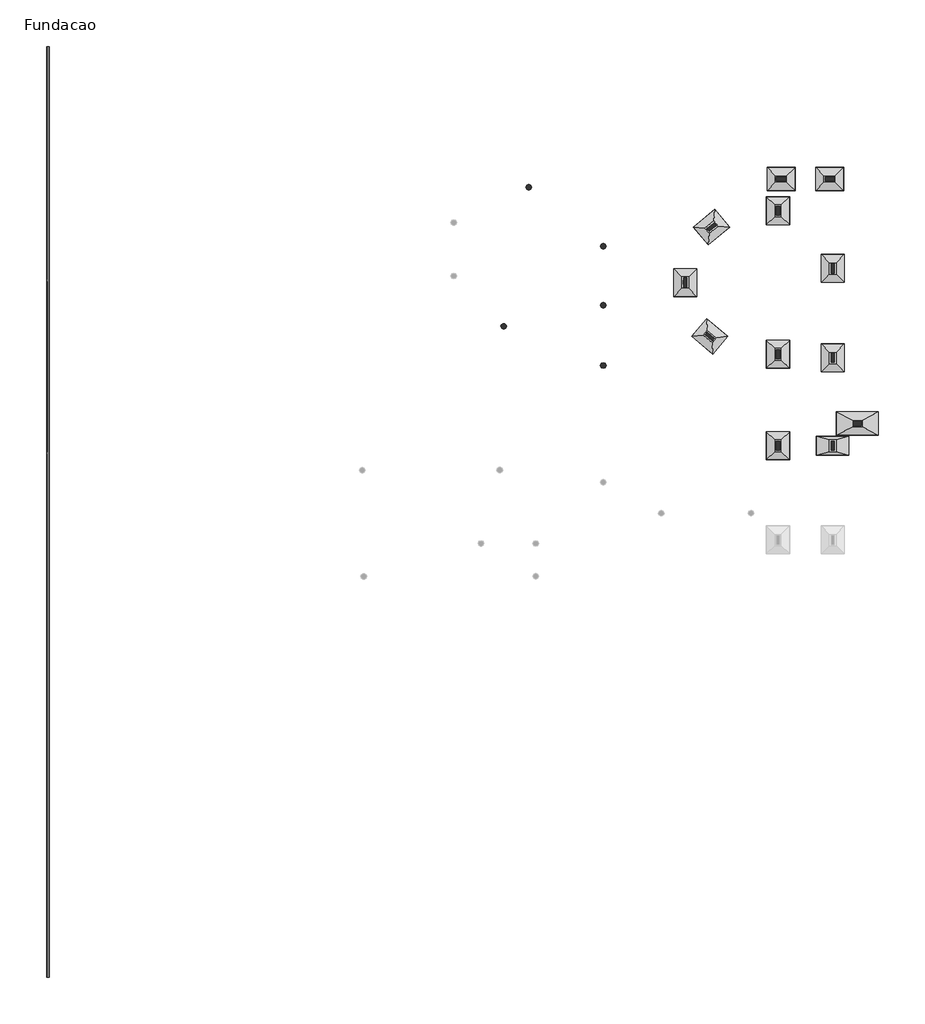
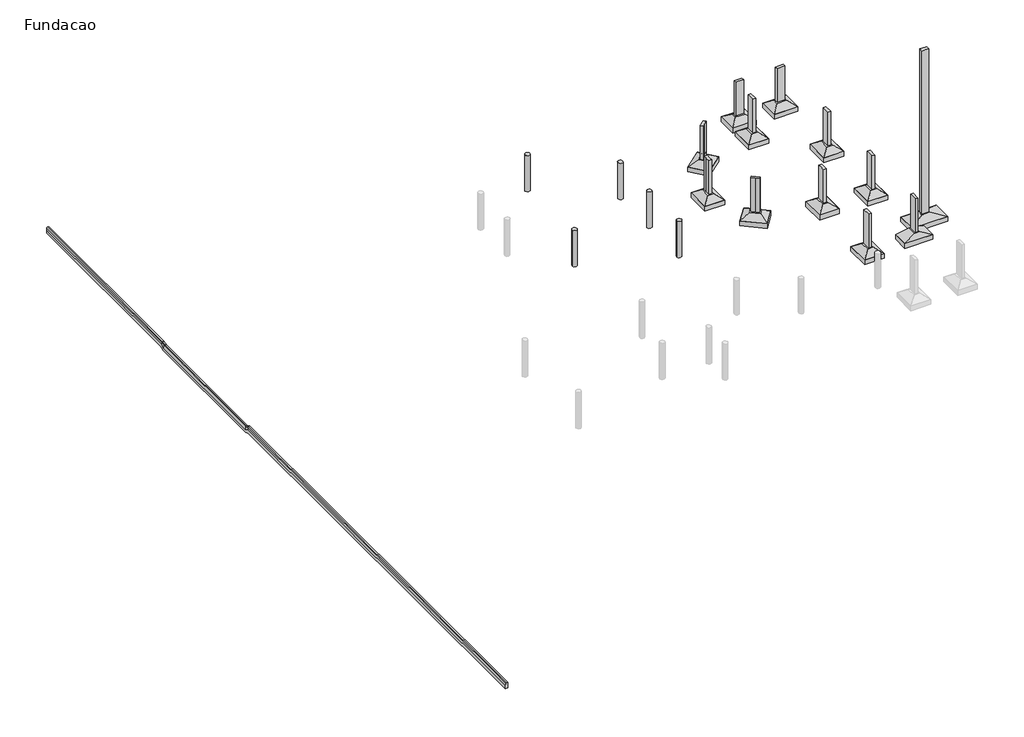
# One storey, part 2 of 2: 17 columns, 12 fasteners, 1 proxy.
"""IFC4 building model written with IfcOpenShell, lengths in millimetres."""

import ifcopenshell
import ifcopenshell.guid

model = None  # the IFC model being written
_history = None  # IfcOwnerHistory: only IFC2X3 demands one
_inside = {}  # id of a spatial element -> (the spatial element, [elements in it])
_under = {}  # id of a project, library or spatial element -> (it, [spatial elements below it])
_declared = {}  # id of a project -> (the project, [libraries it declares])
_typed = {}  # id of a type object -> (the type object, [elements of that type])
_made_of = {}  # id of a material, layer set ... -> (it, [elements and type objects made of it])


def new_model(schema):
    """Start an empty IFC model of exactly this schema.

    Asked for "IFC4X3", IfcOpenShell would pick the latest addendum, in which some entities
    have other attributes; the version numbers below select the first issue.
    IFC2X3 requires an IfcOwnerHistory on every rooted entity: one is made here for all.
    """
    global model, _history
    if schema == "IFC4X3":
        model = ifcopenshell.file(schema_version=(4, 3, 0, 0))
    else:
        model = ifcopenshell.file(schema=schema)
    _inside.clear()
    _under.clear()
    _declared.clear()
    _typed.clear()
    _made_of.clear()
    _history = None
    if model.schema == "IFC2X3":
        org = make("IfcOrganization", Name="unknown")
        user = make(
            "IfcPersonAndOrganization",
            ThePerson=make("IfcPerson", FamilyName="unknown"),
            TheOrganization=org,
        )
        app = make(
            "IfcApplication",
            ApplicationDeveloper=org,
            Version="unknown",
            ApplicationFullName="unknown",
            ApplicationIdentifier="unknown",
        )
        _history = make(
            "IfcOwnerHistory",
            OwningUser=user,
            OwningApplication=app,
            ChangeAction="ADDED",
            CreationDate=0,
        )
    return model


def make(cls, **values):
    """One entity of the class cls with the attributes given. An attribute that is None is left unset."""
    return model.create_entity(
        cls, **{name: value for name, value in values.items() if value is not None}
    )


def rooted(cls, **values):
    """An entity with a GlobalId (a new one), such as an element, a storey or a relation."""
    return make(cls, GlobalId=ifcopenshell.guid.new(), OwnerHistory=_history, **values)


def si_unit(unit_type, name, prefix=None):
    """IfcSIUnit, for example si_unit("LENGTHUNIT", "METRE", prefix="MILLI")."""
    return make("IfcSIUnit", UnitType=unit_type, Prefix=prefix, Name=name)


def assignment(units):
    """IfcUnitAssignment: the units of a project."""
    return None if units is None else make("IfcUnitAssignment", Units=units)


def point(xyz):
    """IfcCartesianPoint."""
    return None if xyz is None else make("IfcCartesianPoint", Coordinates=xyz)


def direction(xyz):
    """IfcDirection."""
    return None if xyz is None else make("IfcDirection", DirectionRatios=xyz)


def frame(location, z_axis=None, x_axis=None):
    """IfcAxis2Placement3D, a coordinate frame: its origin and axes. An axis left out is left unset."""
    return make(
        "IfcAxis2Placement3D",
        Location=point(location),
        Axis=direction(z_axis),
        RefDirection=direction(x_axis),
    )


def origin():
    """The frame at (0, 0, 0) with its axes left unset."""
    return frame((0.0, 0.0, 0.0))


def place(relative_to, where):
    """IfcLocalPlacement: puts the frame where relative to a parent placement (None: the world)."""
    return make(
        "IfcLocalPlacement", PlacementRelTo=relative_to, RelativePlacement=where
    )


def context(
    kind, dimensions, precision=None, world=None, true_north=None, identifier=None
):
    """IfcGeometricRepresentationContext, for example the 3D "Model" context."""
    return make(
        "IfcGeometricRepresentationContext",
        ContextIdentifier=identifier,
        ContextType=kind,
        CoordinateSpaceDimension=dimensions,
        Precision=precision,
        WorldCoordinateSystem=world,
        TrueNorth=true_north,
    )


def project(units=None, contexts=None):
    """IfcProject with its units and contexts."""
    return rooted(
        "IfcProject",
        Name="project",
        RepresentationContexts=contexts,
        UnitsInContext=assignment(units),
    )


def spatial(cls, under=None, at=None, **own):
    """A site, building, storey or space (cls), placed at a placement, below another one or the project."""
    s = rooted(cls, ObjectPlacement=at, **own)
    if under is not None:
        _under.setdefault(under.id(), (under, []))[1].append(s)
    return s


def polyline(points):
    """IfcPolyline through the points."""
    return make("IfcPolyline", Points=[point(p) for p in points])


def circle_curve(where, radius):
    """IfcCircle in the frame where."""
    return make("IfcCircle", Position=where, Radius=radius)


def ellipse_curve(where, semi_axis1, semi_axis2):
    """IfcEllipse in the frame where."""
    return make(
        "IfcEllipse", Position=where, SemiAxis1=semi_axis1, SemiAxis2=semi_axis2
    )


def outline(outer, holes=None, kind="AREA"):
    """IfcArbitraryClosedProfileDef: a profile drawn as a closed curve; with holes, ...WithVoids."""
    if holes is None:
        return make("IfcArbitraryClosedProfileDef", ProfileType=kind, OuterCurve=outer)
    return make(
        "IfcArbitraryProfileDefWithVoids",
        ProfileType=kind,
        OuterCurve=outer,
        InnerCurves=holes,
    )


def extrude(swept, where, along, depth):
    """IfcExtrudedAreaSolid: the profile swept, set in the frame where, extruded along a direction by depth."""
    return make(
        "IfcExtrudedAreaSolid",
        SweptArea=swept,
        Position=where,
        ExtrudedDirection=direction(along),
        Depth=depth,
    )


def faces_of(points, faces, orient=None, outer=None):
    """IfcFace entities. A face is a list of loops; a loop is a list of indices into points, from 0.

    orient and outer hold one flag for each loop. By default every Orientation is true, the
    first loop of a face is its IfcFaceOuterBound and the others are IfcFaceBound.
    """
    made = []
    for i, loops in enumerate(faces):
        bounds = []
        for j, loop in enumerate(loops):
            is_outer = j == 0 if outer is None else outer[i][j]
            bounds.append(
                make(
                    "IfcFaceOuterBound" if is_outer else "IfcFaceBound",
                    Bound=make("IfcPolyLoop", Polygon=[points[k] for k in loop]),
                    Orientation=True if orient is None else orient[i][j],
                )
            )
        made.append(make("IfcFace", Bounds=bounds))
    return made


def faceted_brep(points, faces, orient=None, outer=None, voids=None):
    """IfcFacetedBrep: a solid bounded by flat faces; with voids (closed shells), ...WithVoids."""
    shared = [point(p) for p in points]
    hull = make("IfcClosedShell", CfsFaces=faces_of(shared, faces, orient, outer))
    if voids is None:
        return make("IfcFacetedBrep", Outer=hull)
    return make(
        "IfcFacetedBrepWithVoids",
        Outer=hull,
        Voids=[
            make(cls, CfsFaces=faces_of(shared, fs, o, b)) for cls, fs, o, b in voids
        ],
    )


def shape(context_of_items, identifier, shape_type, items):
    """IfcShapeRepresentation: the items that make up one representation, for example the "Body"."""
    return make(
        "IfcShapeRepresentation",
        ContextOfItems=context_of_items,
        RepresentationIdentifier=identifier,
        RepresentationType=shape_type,
        Items=items,
    )


def source(mapping_origin, context_of_items, identifier, shape_type, items):
    """IfcRepresentationMap: a shape defined once, which mapped items show again and again."""
    return make(
        "IfcRepresentationMap",
        MappingOrigin=mapping_origin,
        MappedRepresentation=shape(context_of_items, identifier, shape_type, items),
    )


def transform(
    local_origin,
    x_axis=None,
    y_axis=None,
    z_axis=None,
    scale=None,
    scale2=None,
    scale3=None,
    uniform=True,
):
    """IfcCartesianTransformationOperator3D, or its non-uniform kind. x_axis, y_axis, z_axis: its Axis1, 2, 3."""
    if uniform:
        return make(
            "IfcCartesianTransformationOperator3D",
            Axis1=direction(x_axis),
            Axis2=direction(y_axis),
            LocalOrigin=point(local_origin),
            Scale=scale,
            Axis3=direction(z_axis),
        )
    return make(
        "IfcCartesianTransformationOperator3DnonUniform",
        Axis1=direction(x_axis),
        Axis2=direction(y_axis),
        LocalOrigin=point(local_origin),
        Scale=scale,
        Axis3=direction(z_axis),
        Scale2=scale2,
        Scale3=scale3,
    )


def mapped(mapping_source, mapping_target):
    """IfcMappedItem: shows the shape of a source again, moved by a transform."""
    return make(
        "IfcMappedItem", MappingSource=mapping_source, MappingTarget=mapping_target
    )


def made_of(thing, what):
    """Note that an element or type object is made of a material, layer set ...; save() writes the relation."""
    if what is not None:
        _made_of.setdefault(what.id(), (what, []))[1].append(thing)
    return thing


def element(
    cls,
    number,
    at=None,
    inside=None,
    cuts=None,
    type_object=None,
    material=None,
    context=None,
    identifier="Body",
    shape_type=None,
    held_by="IfcProductDefinitionShape",
    body=None,
    shapes=None,
    **own,
):
    """One element of the class cls, such as IfcWall. Its Tag is "e" and its number.

    at: its placement. inside: the storey or other place that contains it. cuts: it is an
    opening in that element (IfcRelVoidsElement). A single representation is given by context,
    identifier, shape_type and body (its items); several are given by shapes. held_by: the class
    of the entity that holds the representations. save() writes the other relations.
    """
    e = rooted(cls, Tag="e%d" % number, ObjectPlacement=at, **own)
    if body is not None:
        shapes = [shape(context, identifier, shape_type, body)]
    if shapes is not None:
        e.Representation = make(held_by, Representations=shapes)
    if inside is not None:
        _inside.setdefault(inside.id(), (inside, []))[1].append(e)
    if cuts is not None:
        rooted(
            "IfcRelVoidsElement", RelatingBuildingElement=cuts, RelatedOpeningElement=e
        )
    if type_object is not None:
        _typed.setdefault(type_object.id(), (type_object, []))[1].append(e)
    return made_of(e, material)


def aggregate(whole, parts):
    """IfcRelAggregates: a whole, such as a stair, and the parts it consists of."""
    return rooted("IfcRelAggregates", RelatingObject=whole, RelatedObjects=parts)


def save(model, path):
    """Write the relations noted so far, then the file.

    IfcRelAggregates (storeys below a building ...), IfcRelContainedInSpatialStructure (elements
    in a storey), IfcRelDefinesByType, IfcRelAssociatesMaterial and IfcRelDeclares: one each for
    every whole, place, type object, material and project.
    """
    for whole, parts in _under.values():
        aggregate(whole, parts)
    for where, things in _inside.values():
        rooted(
            "IfcRelContainedInSpatialStructure",
            RelatedElements=things,
            RelatingStructure=where,
        )
    for kind, things in _typed.values():
        rooted("IfcRelDefinesByType", RelatedObjects=things, RelatingType=kind)
    for what, things in _made_of.values():
        rooted("IfcRelAssociatesMaterial", RelatedObjects=things, RelatingMaterial=what)
    for by, libraries in _declared.values():
        rooted("IfcRelDeclares", RelatingContext=by, RelatedDefinitions=libraries)
    model.write(path)


def plane_surface(at):
    """IfcPlane: the flat surface through the origin of the frame at, square to its z axis."""
    return make("IfcPlane", Position=at)


def cylinder_surface(at, radius):
    """IfcCylindricalSurface: all points at the distance radius from the z axis of the frame at."""
    return make("IfcCylindricalSurface", Position=at, Radius=radius)


def advanced_brep(points, edges, surfaces, faces):
    """IfcAdvancedBrep: a solid bounded by faces that lie on surfaces and meet in shared edges.

    An edge is (start, end): straight between two places in points (the first is 0);
    or (start, end, curve); or (start, end, curve, False) where it runs against its curve.
    A face is (place in surfaces, loops), or (place, loops, False) where it looks against
    its surface's normal. A loop lists edges by number (the first is 1), with a minus sign
    where the edge is run from its end to its start. The first loop is the outer one.
    """
    corners = [point(p) for p in points]
    vertices = [make("IfcVertexPoint", VertexGeometry=c) for c in corners]
    made = []
    for start, end, *more in edges:
        made.append(
            make(
                "IfcEdgeCurve",
                EdgeStart=vertices[start],
                EdgeEnd=vertices[end],
                EdgeGeometry=more[0] if more else make("IfcPolyline", Points=[corners[start], corners[end]]),
                SameSense=more[1] if len(more) > 1 else True,
            )
        )
    hull = []
    for where, loops, *sense in faces:
        bounds = []
        for j, loop in enumerate(loops):
            ring = [make("IfcOrientedEdge", EdgeElement=made[abs(k) - 1], Orientation=k > 0) for k in loop]
            bounds.append(
                make(
                    "IfcFaceOuterBound" if j == 0 else "IfcFaceBound",
                    Bound=make("IfcEdgeLoop", EdgeList=ring),
                    Orientation=True,
                )
            )
        hull.append(make("IfcAdvancedFace", Bounds=bounds, FaceSurface=surfaces[where], SameSense=sense[0] if sense else True))
    return make("IfcAdvancedBrep", Outer=make("IfcClosedShell", CfsFaces=hull))


def meio_fio_meio_fio_c5939b1e(model_context):
    return source(origin(), model_context, "Body", "AdvancedBrep", [
        advanced_brep(
        [(-19460.281307, 17327.5225294, 100.0), (-19460.281307, 17327.5225294, -200.0), (-19580.281307, 17327.5225294, -200.0), (-19580.281307, 17327.5225294, -50.0), (-19560.334366, 17327.5225294, 74.7371665), (-19530.7107394, 17327.5225294, 100.0), (-19460.281307, 7304.4300153, 100.0), (-19460.281307, 7104.4300153, 20.0), (-19460.281307, 4.4300153, 20.0), (-19460.281307, -195.5699847, 100.0), (-19460.281307, -22700.938406, 100.0), (-19460.281307, -22700.938406, -200.0), (-19460.281307, -253.3447058, -200.0), (-19460.281307, -53.3447058, -280.0), (-19460.281307, 7162.2047364, -280.0), (-19460.281307, 7362.2047364, -200.0), (-19580.281307, 7362.2047364, -200.0), (-19580.281307, 7162.2047364, -280.0), (-19580.281307, -53.3447058, -280.0), (-19580.281307, -253.3447058, -200.0), (-19580.281307, -22700.938406, -200.0), (-19580.281307, -22700.938406, -50.0), (-19580.281307, -224.4573452, -50.0), (-19580.281307, -24.4573452, -130.0), (-19580.281307, 7133.3173758, -130.0), (-19580.281307, 7333.3173758, -50.0), (-19560.334366, 7309.2951925, 74.7371665), (-19530.7107394, 7304.4300153, 100.0), (-19560.334366, 7109.2951925, -5.2628335), (-19530.7107394, 7104.4300153, 20.0), (-19560.334366, -0.4351619, -5.2628335), (-19530.7107394, 4.4300153, 20.0), (-19560.334366, -200.4351619, 74.7371665), (-19530.7107394, -195.5699847, 100.0), (-19530.7107394, -22700.938406, 100.0), (-19560.334366, -22700.938406, 74.7371665)],
        [
            (0, 1),
            (1, 2),
            (2, 3),
            (3, 4),
            (4, 5, circle_curve(frame((-19530.7107394, 17327.5225294, 70.0), z_axis=(0.0, 1.0, 0.0), x_axis=(-1.0, 0.0, 0.0)), 30.0)),
            (5, 0),
            (0, 6),
            (6, 7),
            (7, 8),
            (8, 9),
            (9, 10),
            (10, 11),
            (11, 12),
            (12, 13),
            (13, 14),
            (14, 15),
            (15, 1),
            (15, 16),
            (16, 2),
            (16, 17),
            (17, 18),
            (18, 19),
            (19, 20),
            (20, 21),
            (21, 22),
            (22, 23),
            (23, 24),
            (24, 25),
            (25, 3),
            (25, 26),
            (26, 4),
            (26, 27, ellipse_curve(frame((-19530.7107394, 7310.2074874, 70.0), z_axis=(0.0, 0.9819563867314226, 0.18910752115494767), x_axis=(0.0, 0.18910752115494667, -0.9819563867314226)), 30.551255, 30.0)),
            (27, 5),
            (27, 6),
            (14, 17),
            (24, 28),
            (28, 26),
            (28, 29, ellipse_curve(frame((-19530.7107394, 7110.2074874, -10.0), z_axis=(0.0, 0.9819563867314226, 0.18910752115494764), x_axis=(0.0, -0.18910752115494842, 0.9819563867314223)), 30.551255, 30.0)),
            (29, 27),
            (29, 7),
            (13, 18),
            (23, 30),
            (30, 28),
            (30, 31, ellipse_curve(frame((-19530.7107394, -1.3474568, -10.0), z_axis=(0.0, 0.9819563867314217, -0.1891075211549513), x_axis=(0.0, 0.18910752115495252, 0.9819563867314217)), 30.551255, 30.0)),
            (31, 29),
            (31, 8),
            (12, 19),
            (22, 32),
            (32, 30),
            (32, 33, ellipse_curve(frame((-19530.7107394, -201.3474568, 70.0), z_axis=(0.0, 0.9819563867314217, -0.18910752115495139), x_axis=(0.0, -0.18910752115495078, -0.9819563867314218)), 30.551255, 30.0)),
            (33, 31),
            (33, 9),
            (10, 34),
            (34, 35, circle_curve(frame((-19530.7107394, -22700.938406, 70.0), z_axis=(0.0, -1.0, 0.0), x_axis=(-1.0, 0.0, 0.0)), 30.0)),
            (35, 21),
            (20, 11),
            (35, 32),
            (34, 33),
        ],
        [
            plane_surface(frame((-19460.281307, 17327.5225294, 100.0), z_axis=(0.0, 1.0, 0.0), x_axis=(0.0, 0.0, 1.0))),
            plane_surface(frame((-19460.281307, 17327.5225294, 100.0), z_axis=(1.0, 0.0, 0.0), x_axis=(0.0, -1.0, 0.0))),
            plane_surface(frame((-19460.281307, 17327.5225294, -200.0), z_axis=(0.0, 0.0, -1.0), x_axis=(0.0, -1.0, 0.0))),
            plane_surface(frame((-19580.281307, 17327.5225294, -200.0), z_axis=(-1.0, 0.0, 0.0), x_axis=(0.0, -1.0, 0.0))),
            plane_surface(frame((-19580.281307, 17327.5225294, -50.0), z_axis=(-0.9874542202157147, 0.0, 0.15790555081495689), x_axis=(0.0, -1.0, 0.0))),
            cylinder_surface(frame((-19530.7107394, 17327.5225294, 70.0), z_axis=(0.0, 1.0, 0.0), x_axis=(-1.0, 0.0, 0.0)), 30.0),
            plane_surface(frame((-19530.7107394, 17327.5225294, 100.0), z_axis=(0.0, 0.0, 1.0), x_axis=(0.0, -1.0, 0.0))),
            plane_surface(frame((-19460.281307, 7362.2047364, -200.0), z_axis=(0.0, 0.3713906763540969, -0.9284766908852621), x_axis=(0.0, -0.9284766908852621, -0.3713906763540969))),
            plane_surface(frame((-19580.281307, 7333.3173758, -50.0), z_axis=(-0.9874542202157147, -0.05864464931723302, 0.1466116232930858), x_axis=(0.0, -0.9284766908852622, -0.3713906763540966))),
            cylinder_surface(frame((-19530.7107394, 7315.5717356, 72.1456993), z_axis=(0.0, 0.9284766908852621, 0.3713906763540969), x_axis=(-1.0, 0.0, 0.0)), 30.0),
            plane_surface(frame((-19530.7107394, 7304.4300153, 100.0), z_axis=(0.0, -0.37139067635409667, 0.9284766908852622), x_axis=(0.0, -0.9284766908852622, -0.37139067635409667))),
            plane_surface(frame((-19460.281307, 7162.2047364, -280.0), z_axis=(0.0, 0.0, -1.0), x_axis=(0.0, -1.0, 0.0))),
            plane_surface(frame((-19580.281307, 7133.3173758, -130.0), z_axis=(-0.9874542202157146, 0.0, 0.15790555081495686), x_axis=(0.0, -1.0, 0.0))),
            cylinder_surface(frame((-19530.7107394, 7104.4300153, -10.0), z_axis=(0.0, 1.0, 0.0), x_axis=(-1.0, 0.0, 0.0)), 30.0),
            plane_surface(frame((-19530.7107394, 7104.4300153, 20.0), z_axis=(0.0, 0.0, 1.0), x_axis=(0.0, -1.0, 0.0))),
            plane_surface(frame((-19460.281307, -53.3447058, -280.0), z_axis=(0.0, -0.37139067635410367, -0.9284766908852594), x_axis=(0.0, -0.9284766908852594, 0.37139067635410367))),
            plane_surface(frame((-19580.281307, -24.4573452, -130.0), z_axis=(-0.9874542202157147, 0.05864464931723411, 0.14661162329308536), x_axis=(0.0, -0.9284766908852594, 0.37139067635410355))),
            cylinder_surface(frame((-19530.7107394, -6.711705, -7.8543007), z_axis=(0.0, 0.9284766908852593, -0.3713906763541038), x_axis=(-1.0, 0.0, 0.0)), 30.0),
            plane_surface(frame((-19530.7107394, 4.4300153, 20.0), z_axis=(0.0, 0.3713906763541038, 0.9284766908852593), x_axis=(0.0, -0.9284766908852593, 0.3713906763541038))),
            plane_surface(frame((-19460.281307, -22700.938406, 100.0), z_axis=(0.0, -1.0, 0.0), x_axis=(0.0, 0.0, 1.0))),
            plane_surface(frame((-19460.281307, -253.3447058, -200.0), z_axis=(0.0, 0.0, -1.0), x_axis=(0.0, -1.0, 0.0))),
            plane_surface(frame((-19580.281307, -224.4573452, -50.0), z_axis=(-0.9874542202157146, 0.0, 0.15790555081495683), x_axis=(0.0, -1.0, 0.0))),
            cylinder_surface(frame((-19530.7107394, -195.5699847, 70.0), z_axis=(0.0, 1.0, 0.0), x_axis=(-1.0, 0.0, 0.0)), 30.0),
            plane_surface(frame((-19530.7107394, -195.5699847, 100.0), z_axis=(0.0, 0.0, 1.0), x_axis=(0.0, -1.0, 0.0))),
        ],
        [
            (0, [[1, 2, 3, 4, 5, 6]]),
            (1, [[-1, 7, 8, 9, 10, 11, 12, 13, 14, 15, 16, 17]]),
            (2, [[-2, -17, 18, 19]]),
            (3, [[-3, -19, 20, 21, 22, 23, 24, 25, 26, 27, 28, 29]]),
            (4, [[-4, -29, 30, 31]]),
            (5, [[-5, -31, 32, 33]]),
            (6, [[-6, -33, 34, -7]]),
            (7, [[-18, -16, 35, -20]]),
            (8, [[-30, -28, 36, 37]]),
            (9, [[-32, -37, 38, 39]]),
            (10, [[-34, -39, 40, -8]]),
            (11, [[-35, -15, 41, -21]]),
            (12, [[-36, -27, 42, 43]]),
            (13, [[-38, -43, 44, 45]]),
            (14, [[-40, -45, 46, -9]]),
            (15, [[-41, -14, 47, -22]]),
            (16, [[-42, -26, 48, 49]]),
            (17, [[-44, -49, 50, 51]]),
            (18, [[-46, -51, 52, -10]]),
            (19, [[53, 54, 55, -24, 56, -12]]),
            (20, [[-47, -13, -56, -23]]),
            (21, [[-48, -25, -55, 57]]),
            (22, [[-50, -57, -54, 58]]),
            (23, [[-52, -58, -53, -11]]),
        ],
    ),
    ])


def s14_8166d2be(model_context):
    return source(origin(), model_context, "Body", "SolidModel", [
        faceted_brep([(-55.0, 0.0, 0.0), (-345.0, 0.0, 0.0), (-345.0, -400.0, 0.0), (-55.0, -400.0, 0.0), (300.0, 700.0, -250.0), (300.0, -1100.0, -250.0), (-700.0, -1100.0, -250.0), (-700.0, 700.0, -250.0)], [[[0, 1, 2, 3]], [[4, 5, 6, 7]], [[4, 7, 1, 0]], [[7, 6, 2, 1]], [[6, 5, 3, 2]], [[5, 4, 0, 3]]]),
        extrude(outline(polyline([(300.0, 700.0), (300.0, -1100.0), (-700.0, -1100.0), (-700.0, 700.0), (300.0, 700.0)])), frame((0.0, 0.0, -500.0), z_axis=(0.0, 0.0, 1.0), x_axis=(1.0, 0.0, 0.0)), (0.0, 0.0, 1.0), 250.0),
    ])


def sps1_6b3be553(model_context):
    return source(origin(), model_context, "Body", "SolidModel", [
        faceted_brep([(-55.0, 50.0, 0.0), (-345.0, 50.0, 0.0), (-345.0, -450.0, 0.0), (-55.0, -450.0, 0.0), (300.0, 400.0, -250.0), (300.0, -800.0, -250.0), (-700.0, -800.0, -250.0), (-700.0, 400.0, -250.0)], [[[0, 1, 2, 3]], [[4, 5, 6, 7]], [[4, 7, 1, 0]], [[7, 6, 2, 1]], [[6, 5, 3, 2]], [[5, 4, 0, 3]]]),
        extrude(outline(polyline([(300.0, 400.0), (300.0, -800.0), (-700.0, -800.0), (-700.0, 400.0), (300.0, 400.0)])), frame((0.0, 0.0, -500.0), z_axis=(0.0, 0.0, 1.0), x_axis=(1.0, 0.0, 0.0)), (0.0, 0.0, 1.0), 250.0),
    ])


def sps11_3ae28187(model_context):
    return source(origin(), model_context, "Body", "SolidModel", [
        faceted_brep([(-55.0, 50.0, 0.0), (-345.0, 50.0, 0.0), (-345.0, -450.0, 0.0), (-55.0, -450.0, 0.0), (500.0, 200.0, -250.0), (500.0, -600.0, -250.0), (-900.0, -600.0, -250.0), (-900.0, 200.0, -250.0)], [[[0, 1, 2, 3]], [[4, 5, 6, 7]], [[4, 7, 1, 0]], [[7, 6, 2, 1]], [[6, 5, 3, 2]], [[5, 4, 0, 3]]]),
        extrude(outline(polyline([(500.0, 200.0), (500.0, -600.0), (-900.0, -600.0), (-900.0, 200.0), (500.0, 200.0)])), frame((0.0, 0.0, -500.0), z_axis=(0.0, 0.0, 1.0), x_axis=(1.0, 0.0, 0.0)), (0.0, 0.0, 1.0), 250.0),
    ])


model = new_model("IFC4")

# Units and contexts
model_context = context("Model", 3, world=origin())
ifc_project = project(units=[si_unit("LENGTHUNIT", "METRE", prefix="MILLI")], contexts=[model_context])

# Site, building, storey
site = spatial("IfcSite", under=ifc_project)
building = spatial("IfcBuilding", under=site)
storey = spatial("IfcBuildingStorey", under=building, Name="Fundacao", Elevation=-1200.0)

# Proxy
placement = place(None, origin())
meio_fio_meio_fio_shape = meio_fio_meio_fio_c5939b1e(model_context)
element("IfcBuildingElementProxy", 1, Name="MEIO-FIO : MEIO-FIO", ObjectType="MEIO-FIO : MEIO-FIO", at=placement, inside=storey, context=model_context, shape_type="MappedRepresentation", body=[
    mapped(meio_fio_meio_fio_shape, transform((0.0, 0.0, 0.0), x_axis=(1.0, 0.0, 0.0), y_axis=(0.0, 1.0, 0.0), z_axis=(0.0, 0.0, 1.0))),
])

# Columns
element("IfcColumn", 2, ObjectType="TQS - Pilar circular : TQS - Pilar circular 25.0cm", at=placement, inside=storey, context=model_context, shape_type="AdvancedBrep", body=[
    advanced_brep(
    [(-51.2, 5294.463685, -1500.0), (198.8, 5294.463685, -1500.0), (-51.2, 5294.463685, 430.0), (198.8, 5294.463685, 430.0), (143.8, 5190.9021092, 430.0), (3.8, 5190.9021092, 430.0)],
    [
        (0, 1, circle_curve(frame((73.8, 5294.463685, -1500.0), z_axis=(0.0, 0.0, -1.0), x_axis=(1.0, 0.0, 0.0)), 125.0)),
        (1, 0, circle_curve(frame((73.8, 5294.463685, -1500.0), z_axis=(0.0, 0.0, -1.0), x_axis=(1.0, 0.0, 0.0)), 125.0)),
        (2, 3, circle_curve(frame((73.8, 5294.463685, 430.0), z_axis=(0.0, 0.0, -1.0), x_axis=(1.0, 0.0, 0.0)), 125.0)),
        (3, 1),
        (0, 2),
        (3, 4, circle_curve(frame((73.8, 5294.463685, 430.0), z_axis=(0.0, 0.0, -1.0), x_axis=(1.0, 0.0, 0.0)), 125.0)),
        (4, 5, circle_curve(frame((73.8, 5294.463685, 430.0), z_axis=(0.0, 0.0, -1.0), x_axis=(1.0, 0.0, 0.0)), 125.0)),
        (5, 2, circle_curve(frame((73.8, 5294.463685, 430.0), z_axis=(0.0, 0.0, -1.0), x_axis=(1.0, 0.0, 0.0)), 125.0)),
    ],
    [
        plane_surface(frame((198.8, 5294.463685, -1500.0), z_axis=(0.0, 0.0, -1.0), x_axis=(0.0, -1.0, 0.0))),
        cylinder_surface(frame((73.8, 5294.463685, -1500.0), z_axis=(0.0, 0.0, 1.0), x_axis=(1.0, 0.0, 0.0)), 125.0),
        plane_surface(frame((198.8, 5294.463685, 430.0), z_axis=(0.0, 0.0, 1.0), x_axis=(0.0, 1.0, 0.0))),
    ],
    [
        (0, [[1, 2]]),
        (1, [[3, 4, -1, 5]]),
        (1, [[6, 7, 8, -5, -2, -4]]),
        (2, [[-8, -7, -6, -3]]),
    ],
),
])
element("IfcColumn", 3, ObjectType="TQS - Pilar circular : TQS - Pilar circular 25.0cm", at=placement, inside=storey, context=model_context, shape_type="AdvancedBrep", body=[
    advanced_brep(
    [(1025.0, 11273.8, -1500.0), (1275.0, 11273.8, -1500.0), (1025.0, 11273.8, 430.0), (1068.781362, 11368.818592, 430.0), (1231.240384, 11368.8, 430.0), (1275.0, 11273.8, 430.0), (1231.240384, 11178.8, 430.0), (1068.781362, 11178.781408, 430.0)],
    [
        (0, 1, circle_curve(frame((1150.0, 11273.8, -1500.0), z_axis=(0.0, 0.0, -1.0), x_axis=(1.0, 0.0, 0.0)), 125.0)),
        (1, 0, circle_curve(frame((1150.0, 11273.8, -1500.0), z_axis=(0.0, 0.0, -1.0), x_axis=(1.0, 0.0, 0.0)), 125.0)),
        (2, 3, circle_curve(frame((1150.0, 11273.8, 430.0), z_axis=(0.0, 0.0, -1.0), x_axis=(1.0, 0.0, 0.0)), 125.0)),
        (3, 4, circle_curve(frame((1150.0, 11273.8, 430.0), z_axis=(0.0, 0.0, -1.0), x_axis=(1.0, 0.0, 0.0)), 125.0)),
        (4, 5, circle_curve(frame((1150.0, 11273.8, 430.0), z_axis=(0.0, 0.0, -1.0), x_axis=(1.0, 0.0, 0.0)), 125.0)),
        (5, 1),
        (0, 2),
        (5, 6, circle_curve(frame((1150.0, 11273.8, 430.0), z_axis=(0.0, 0.0, -1.0), x_axis=(1.0, 0.0, 0.0)), 125.0)),
        (6, 7, circle_curve(frame((1150.0, 11273.8, 430.0), z_axis=(0.0, 0.0, -1.0), x_axis=(1.0, 0.0, 0.0)), 125.0)),
        (7, 2, circle_curve(frame((1150.0, 11273.8, 430.0), z_axis=(0.0, 0.0, -1.0), x_axis=(1.0, 0.0, 0.0)), 125.0)),
    ],
    [
        plane_surface(frame((1275.0, 11273.8, -1500.0), z_axis=(0.0, 0.0, -1.0), x_axis=(0.0, -1.0, 0.0))),
        cylinder_surface(frame((1150.0, 11273.8, -1500.0), z_axis=(0.0, 0.0, 1.0), x_axis=(1.0, 0.0, 0.0)), 125.0),
        plane_surface(frame((1275.0, 11273.8, 430.0), z_axis=(0.0, 0.0, 1.0), x_axis=(0.0, 1.0, 0.0))),
    ],
    [
        (0, [[1, 2]]),
        (1, [[3, 4, 5, 6, -1, 7]]),
        (1, [[8, 9, 10, -7, -2, -6]]),
        (2, [[-10, -9, -8, -5, -4, -3]]),
    ],
),
])
element("IfcColumn", 4, ObjectType="TQS - Pilar circular : TQS - Pilar circular 25.0cm", at=placement, inside=storey, context=model_context, shape_type="AdvancedBrep", body=[
    advanced_brep(
    [(4239.0, 6198.7999999, -1500.0), (4489.0, 6198.7999999, -1500.0), (4239.0, 6198.7999999, 430.0), (4269.0, 6280.040384, 430.0), (4459.0, 6280.040384, 430.0), (4489.0, 6198.7999999, 430.0), (4459.0, 6117.5596159, 430.0), (4269.0, 6117.5596159, 430.0)],
    [
        (0, 1, circle_curve(frame((4364.0, 6198.7999999, -1500.0), z_axis=(0.0, 0.0, -1.0), x_axis=(1.0, 0.0, 0.0)), 125.0)),
        (1, 0, circle_curve(frame((4364.0, 6198.7999999, -1500.0), z_axis=(0.0, 0.0, -1.0), x_axis=(1.0, 0.0, 0.0)), 125.0)),
        (2, 3, circle_curve(frame((4364.0, 6198.7999999, 430.0), z_axis=(0.0, 0.0, -1.0), x_axis=(1.0, 0.0, 0.0)), 125.0)),
        (3, 4, circle_curve(frame((4364.0, 6198.7999999, 430.0), z_axis=(0.0, 0.0, -1.0), x_axis=(1.0, 0.0, 0.0)), 125.0)),
        (4, 5, circle_curve(frame((4364.0, 6198.7999999, 430.0), z_axis=(0.0, 0.0, -1.0), x_axis=(1.0, 0.0, 0.0)), 125.0)),
        (5, 1),
        (0, 2),
        (5, 6, circle_curve(frame((4364.0, 6198.7999999, 430.0), z_axis=(0.0, 0.0, -1.0), x_axis=(1.0, 0.0, 0.0)), 125.0)),
        (6, 7, circle_curve(frame((4364.0, 6198.7999999, 430.0), z_axis=(0.0, 0.0, -1.0), x_axis=(1.0, 0.0, 0.0)), 125.0)),
        (7, 2, circle_curve(frame((4364.0, 6198.7999999, 430.0), z_axis=(0.0, 0.0, -1.0), x_axis=(1.0, 0.0, 0.0)), 125.0)),
    ],
    [
        plane_surface(frame((4489.0, 6198.7999999, -1500.0), z_axis=(0.0, 0.0, -1.0), x_axis=(0.0, -1.0, 0.0))),
        cylinder_surface(frame((4364.0, 6198.7999999, -1500.0), z_axis=(0.0, 0.0, 1.0), x_axis=(1.0, 0.0, 0.0)), 125.0),
        plane_surface(frame((4489.0, 6198.7999999, 430.0), z_axis=(0.0, 0.0, 1.0), x_axis=(0.0, 1.0, 0.0))),
    ],
    [
        (0, [[1, 2]]),
        (1, [[3, 4, 5, 6, -1, 7]]),
        (1, [[8, 9, 10, -7, -2, -6]]),
        (2, [[-10, -9, -8, -5, -4, -3]]),
    ],
),
])
element("IfcColumn", 5, ObjectType="TQS - Pilar circular : TQS - Pilar circular 25.0cm", at=placement, inside=storey, context=model_context, shape_type="AdvancedBrep", body=[
    advanced_brep(
    [(4239.0, 8736.2999999, -1500.0), (4489.0, 8736.2999999, -1500.0), (4239.0, 8736.2999999, 430.0), (4269.0, 8817.540384, 430.0), (4459.0, 8817.540384, 430.0), (4489.0, 8736.2999999, 430.0), (4459.0, 8655.0596159, 430.0), (4269.0, 8655.0596159, 430.0)],
    [
        (0, 1, circle_curve(frame((4364.0, 8736.2999999, -1500.0), z_axis=(0.0, 0.0, -1.0), x_axis=(1.0, 0.0, 0.0)), 125.0)),
        (1, 0, circle_curve(frame((4364.0, 8736.2999999, -1500.0), z_axis=(0.0, 0.0, -1.0), x_axis=(1.0, 0.0, 0.0)), 125.0)),
        (2, 3, circle_curve(frame((4364.0, 8736.2999999, 430.0), z_axis=(0.0, 0.0, -1.0), x_axis=(1.0, 0.0, 0.0)), 125.0)),
        (3, 4, circle_curve(frame((4364.0, 8736.2999999, 430.0), z_axis=(0.0, 0.0, -1.0), x_axis=(1.0, 0.0, 0.0)), 125.0)),
        (4, 5, circle_curve(frame((4364.0, 8736.2999999, 430.0), z_axis=(0.0, 0.0, -1.0), x_axis=(1.0, 0.0, 0.0)), 125.0)),
        (5, 1),
        (0, 2),
        (5, 6, circle_curve(frame((4364.0, 8736.2999999, 430.0), z_axis=(0.0, 0.0, -1.0), x_axis=(1.0, 0.0, 0.0)), 125.0)),
        (6, 7, circle_curve(frame((4364.0, 8736.2999999, 430.0), z_axis=(0.0, 0.0, -1.0), x_axis=(1.0, 0.0, 0.0)), 125.0)),
        (7, 2, circle_curve(frame((4364.0, 8736.2999999, 430.0), z_axis=(0.0, 0.0, -1.0), x_axis=(1.0, 0.0, 0.0)), 125.0)),
    ],
    [
        plane_surface(frame((4489.0, 8736.2999999, -1500.0), z_axis=(0.0, 0.0, -1.0), x_axis=(0.0, -1.0, 0.0))),
        cylinder_surface(frame((4364.0, 8736.2999999, -1500.0), z_axis=(0.0, 0.0, 1.0), x_axis=(1.0, 0.0, 0.0)), 125.0),
        plane_surface(frame((4489.0, 8736.2999999, 430.0), z_axis=(0.0, 0.0, 1.0), x_axis=(0.0, 1.0, 0.0))),
    ],
    [
        (0, [[1, 2]]),
        (1, [[3, 4, 5, 6, -1, 7]]),
        (1, [[8, 9, 10, -7, -2, -6]]),
        (2, [[-10, -9, -8, -5, -4, -3]]),
    ],
),
])
element("IfcColumn", 6, ObjectType="TQS - Pilar circular : TQS - Pilar circular 25.0cm", at=placement, inside=storey, context=model_context, shape_type="AdvancedBrep", body=[
    advanced_brep(
    [(4239.0, 3610.8, -1500.0), (4489.0, 3610.8, -1500.0), (4239.0, 3610.8, 430.0), (4269.0, 3692.040384, 430.0), (4459.0, 3692.040384, 430.0), (4489.0, 3610.8, 430.0), (4459.0, 3529.5596159, 430.0), (4269.0, 3529.5596159, 430.0)],
    [
        (0, 1, circle_curve(frame((4364.0, 3610.8, -1500.0), z_axis=(0.0, 0.0, -1.0), x_axis=(1.0, 0.0, 0.0)), 125.0)),
        (1, 0, circle_curve(frame((4364.0, 3610.8, -1500.0), z_axis=(0.0, 0.0, -1.0), x_axis=(1.0, 0.0, 0.0)), 125.0)),
        (2, 3, circle_curve(frame((4364.0, 3610.8, 430.0), z_axis=(0.0, 0.0, -1.0), x_axis=(1.0, 0.0, 0.0)), 125.0)),
        (3, 4, circle_curve(frame((4364.0, 3610.8, 430.0), z_axis=(0.0, 0.0, -1.0), x_axis=(1.0, 0.0, 0.0)), 125.0)),
        (4, 5, circle_curve(frame((4364.0, 3610.8, 430.0), z_axis=(0.0, 0.0, -1.0), x_axis=(1.0, 0.0, 0.0)), 125.0)),
        (5, 1),
        (0, 2),
        (5, 6, circle_curve(frame((4364.0, 3610.8, 430.0), z_axis=(0.0, 0.0, -1.0), x_axis=(1.0, 0.0, 0.0)), 125.0)),
        (6, 7, circle_curve(frame((4364.0, 3610.8, 430.0), z_axis=(0.0, 0.0, -1.0), x_axis=(1.0, 0.0, 0.0)), 125.0)),
        (7, 2, circle_curve(frame((4364.0, 3610.8, 430.0), z_axis=(0.0, 0.0, -1.0), x_axis=(1.0, 0.0, 0.0)), 125.0)),
    ],
    [
        plane_surface(frame((4489.0, 3610.8, -1500.0), z_axis=(0.0, 0.0, -1.0), x_axis=(0.0, -1.0, 0.0))),
        cylinder_surface(frame((4364.0, 3610.8, -1500.0), z_axis=(0.0, 0.0, 1.0), x_axis=(1.0, 0.0, 0.0)), 125.0),
        plane_surface(frame((4489.0, 3610.8, 430.0), z_axis=(0.0, 0.0, 1.0), x_axis=(0.0, 1.0, 0.0))),
    ],
    [
        (0, [[1, 2]]),
        (1, [[3, 4, 5, 6, -1, 7]]),
        (1, [[8, 9, 10, -7, -2, -6]]),
        (2, [[-10, -9, -8, -5, -4, -3]]),
    ],
),
])
element("IfcColumn", 7, ObjectType="TQS - Pilar retangular : 14.0 x 40.0", at=placement, inside=storey, context=model_context, shape_type="Brep", body=[
    faceted_brep([(14294.0, 11563.8, -1450.0), (14154.0, 11563.8, -1450.0), (13894.0, 11563.8, -1450.0), (13894.0, 11703.8, -1450.0), (14294.0, 11703.8, -1450.0), (14294.0, 11563.8, 350.0), (14154.0, 11563.8, 350.0), (13894.0, 11563.8, 350.0), (13894.0, 11703.8, 350.0), (14294.0, 11703.8, 350.0)], [[[0, 1, 2, 3, 4]], [[5, 6, 7, 2, 1, 0]], [[7, 8, 3, 2]], [[8, 9, 4, 3]], [[9, 5, 0, 4]], [[5, 9, 8, 7, 6]]]),
])
element("IfcColumn", 8, ObjectType="TQS - Pilar retangular : 14.0 x 40.0", at=placement, inside=storey, context=model_context, shape_type="Brep", body=[
    faceted_brep([(12206.0, 11563.8, -1450.0), (11946.0031341, 11563.8, -1450.0), (11806.0, 11563.8, -1450.0), (11806.0, 11703.8, -1450.0), (12206.0, 11703.8, -1450.0), (12206.0, 11563.8, 350.0), (11946.0031341, 11563.8, 350.0), (11806.0, 11563.8, 350.0), (11806.0, 11703.8, 350.0), (12206.0, 11703.8, 350.0)], [[[0, 1, 2, 3, 4]], [[5, 6, 7, 2, 1, 0]], [[7, 8, 3, 2]], [[8, 9, 4, 3]], [[9, 5, 0, 4]], [[5, 9, 8, 7, 6]]]),
])
element("IfcColumn", 9, ObjectType="TQS - Pilar retangular : 14.0 x 40.0", at=placement, inside=storey, context=model_context, shape_type="Brep", body=[
    faceted_brep([(11806.0031341, 10065.0703526, -1450.0), (11806.0031341, 10209.2668795, -1450.0), (11806.0031341, 10465.0703526, -1450.0), (11946.0031341, 10465.0703526, -1450.0), (11946.0031341, 10065.0703526, -1450.0), (11806.0031341, 10065.0703526, -1250.0), (11806.0031341, 10065.0703526, 350.0), (11806.0031341, 10209.2668795, 350.0), (11806.0031341, 10465.0703526, 350.0), (11946.0031341, 10465.0703526, 350.0), (11946.0031341, 10465.0703526, -1250.0), (11946.0031341, 10065.0703526, 350.0), (11946.0031341, 10065.0703526, -1250.0)], [[[0, 1, 2, 3, 4]], [[2, 1, 0, 5, 6, 7, 8]], [[3, 2, 8, 9, 10]], [[4, 3, 10, 9, 11, 12]], [[0, 4, 12, 11, 6, 5]], [[8, 7, 6, 11, 9]]]),
])
element("IfcColumn", 10, ObjectType="TQS - Pilar retangular : 14.0 x 40.0", at=placement, inside=storey, context=model_context, shape_type="Brep", body=[
    faceted_brep([(11806.0, 3898.2763649, -1450.0), (11806.0, 4154.0974781, -1450.0), (11806.0, 4298.2763649, -1450.0), (11946.0, 4298.2763649, -1450.0), (11946.0, 3898.2763649, -1450.0), (11806.0, 3898.2763649, 350.0), (11806.0, 4154.0974781, 350.0), (11806.0, 4298.2763649, 350.0), (11806.0, 4298.2763649, -1250.0), (11946.0, 4298.2763649, 350.0), (11946.0, 4298.2763649, -1250.0), (11946.0, 3898.2763649, 350.0), (11946.0, 3898.2763649, -1250.0)], [[[0, 1, 2, 3, 4]], [[2, 1, 0, 5, 6, 7, 8]], [[3, 2, 8, 7, 9, 10]], [[4, 3, 10, 9, 11, 12]], [[0, 4, 12, 11, 5]], [[7, 6, 5, 11, 9]]]),
])
element("IfcColumn", 11, ObjectType="TQS - Pilar retangular : 14.0 x 40.0", at=placement, inside=storey, context=model_context, shape_type="Brep", body=[
    faceted_brep([(11806.0, -35.7794604, -1450.0), (11806.0, 364.2205396, -1450.0), (11946.0, 364.2205396, -1450.0), (11946.0, -35.7794604, -1450.0), (11806.0, -35.7794604, 350.0), (11806.0, 364.2205396, 350.0), (11946.0, 364.2205396, 350.0), (11946.0, 364.2205396, -1250.0), (11946.0, -35.7794604, 350.0), (11946.0, -35.7794604, -1250.0)], [[[0, 1, 2, 3]], [[1, 0, 4, 5]], [[2, 1, 5, 6, 7]], [[3, 2, 7, 6, 8, 9]], [[0, 3, 9, 8, 4]], [[5, 4, 8, 6]]]),
])
element("IfcColumn", 12, ObjectType="TQS - Pilar retangular : 14.0 x 40.0", at=placement, inside=storey, context=model_context, shape_type="SweptSolid", body=[
    extrude(outline(polyline([(14154.0, -35.7794604), (14154.0, 364.2205396), (14294.0, 364.2205396), (14294.0, -35.7794604), (14154.0, -35.7794604)])), frame((0.0, 0.0, -1450.0), z_axis=(0.0, 0.0, 1.0), x_axis=(1.0, 0.0, 0.0)), (0.0, 0.0, 1.0), 1800.0),
])
element("IfcColumn", 13, ObjectType="TQS - Pilar retangular : 14.0 x 40.0", at=placement, inside=storey, context=model_context, shape_type="SweptSolid", body=[
    extrude(outline(polyline([(14154.0, 3742.9688701), (14154.0, 4142.9688701), (14294.0, 4142.9688701), (14294.0, 3742.9688701), (14154.0, 3742.9688701)])), frame((0.0, 0.0, -1450.0), z_axis=(0.0, 0.0, 1.0), x_axis=(1.0, 0.0, 0.0)), (0.0, 0.0, 1.0), 1800.0),
])
element("IfcColumn", 14, ObjectType="TQS - Pilar retangular : 14.0 x 40.0", at=placement, inside=storey, context=model_context, shape_type="SweptSolid", body=[
    extrude(outline(polyline([(14154.0, 7588.3844351), (14154.0, 7988.3844351), (14294.0, 7988.3844351), (14294.0, 7588.3844351), (14154.0, 7588.3844351)])), frame((0.0, 0.0, -1450.0), z_axis=(0.0, 0.0, 1.0), x_axis=(1.0, 0.0, 0.0)), (0.0, 0.0, 1.0), 1800.0),
])
element("IfcColumn", 15, ObjectType="TQS - Pilar retangular : 19.0 x 35.0", at=placement, inside=storey, context=model_context, shape_type="Brep", body=[
    faceted_brep([(15109.0, 1218.8, -1450.0), (15459.0, 1218.8, -1450.0), (15459.0, 1028.8, -1450.0), (15109.0, 1028.8, -1450.0), (15109.0, 1218.8, 7250.0), (15459.0, 1218.8, 7250.0), (15109.0, 1218.8, 3030.0), (15109.0, 1218.8, 3530.0), (15459.0, 1028.8, 7250.0), (15459.0, 1028.8, 6450.0), (15459.0, 1028.8, 3530.0), (15459.0, 1028.8, 3030.0), (15269.0, 1028.8, 7250.0), (15109.0, 1028.8, 7250.0), (15109.0, 1028.8, 3530.0), (15109.0, 1028.8, 3030.0)], [[[0, 1, 2, 3]], [[4, 5, 1, 0, 6, 7]], [[5, 8, 9, 10, 11, 2, 1]], [[8, 12, 13, 14, 15, 3, 2, 11, 10, 9]], [[13, 4, 7, 6, 0, 3, 15, 14]], [[4, 13, 12, 8, 5]]]),
])
element("IfcColumn", 16, ObjectType="TQS - Pilar Polig_1 : TQS Column", at=placement, inside=storey, context=model_context, shape_type="Brep", body=[
    faceted_brep([(8972.0852614, 9622.0701515, -1450.0), (8976.3671199, 9625.3602237, -1450.0), (9127.4604175, 9741.4565052, -1450.0), (9213.935877, 9632.7302414, -1450.0), (9057.0815461, 9512.0930505, -1450.0), (8905.0139036, 9380.7810997, -1450.0), (8818.2678219, 9491.8005445, -1450.0), (8817.5300259, 9492.7447911, -1450.0), (8829.0985229, 9502.4248258, -1450.0), (8972.0852614, 9622.0701515, 350.0), (8976.3671199, 9625.3602237, 350.0), (9127.4604175, 9741.4565052, 350.0), (9214.7474586, 9631.7098337, 350.0), (9214.7474586, 9631.7098337, -1250.0), (9213.935877, 9632.7302414, -1250.0), (9057.0815461, 9512.0930505, 350.0), (9057.0815461, 9512.0930505, -1250.0), (8905.5686682, 9380.0711005, 350.0), (8905.5686682, 9380.0711005, -1250.0), (8905.0139036, 9380.7810997, 350.0), (8818.2678219, 9491.8005445, 350.0), (8817.5300259, 9492.7447911, 350.0), (8905.0139036, 9380.7810997, -1250.0), (8829.0985229, 9502.4248258, 350.0)], [[[0, 1, 2, 3, 4, 5, 6, 7, 8]], [[2, 1, 0, 9, 10, 11]], [[2, 11, 12, 13, 14, 3]], [[12, 15, 16, 13]], [[15, 17, 18, 16]], [[17, 19, 20, 21, 7, 6, 5, 22, 18]], [[0, 8, 7, 21, 23, 9]], [[11, 10, 9, 23, 21, 20, 19, 17, 15, 12]], [[16, 14, 13]], [[16, 22, 5, 4]], [[14, 16, 4, 3]], [[22, 16, 18]]]),
])
element("IfcColumn", 17, ObjectType="TQS - Pilar Polig_1 : TQS Column", at=placement, inside=storey, context=model_context, shape_type="Brep", body=[
    faceted_brep([(7807.1607904, 7184.6059928, -1450.0), (7813.3909991, 7380.4521699, -1450.0), (7952.8314751, 7378.3521249, -1450.0), (7953.6012, 7378.3405325, -1450.0), (7946.0963828, 7180.5770563, -1450.0), (7952.0851569, 6979.7037579, -1450.0), (7809.1351911, 6983.0905557, -1450.0), (7807.2096878, 7179.6153242, -1450.0), (7807.1607904, 7184.6059928, 350.0), (7813.3909991, 7380.4521699, 350.0), (7952.8314751, 7378.3521249, 350.0), (7953.6012, 7378.3405325, 350.0), (7946.0963828, 7180.5770563, 350.0), (7952.0851569, 6979.7037579, 350.0), (7809.1351911, 6983.0905557, 350.0), (7807.2096878, 7179.6153242, 350.0)], [[[0, 1, 2, 3, 4, 5, 6, 7]], [[8, 9, 1, 0]], [[9, 10, 11, 3, 2, 1]], [[11, 12, 4, 3]], [[12, 13, 5, 4]], [[13, 14, 6, 5]], [[14, 15, 8, 0, 7, 6]], [[8, 15, 14, 13, 12, 11, 10, 9]]]),
])
element("IfcColumn", 18, ObjectType="TQS - Pilar Polig_2 : TQS Column", at=placement, inside=storey, context=model_context, shape_type="Brep", body=[
    faceted_brep([(8896.4640317, 4801.2041983, -1450.0), (8741.5682427, 4944.2508424, -1450.0), (8835.150532, 5048.5754434, -1450.0), (8986.5977359, 4908.3461751, -1450.0), (9137.421848, 4786.4870592, -1450.0), (9137.2576489, 4786.3047048, -1450.0), (9043.2613751, 4681.915321, -1450.0), (8896.4640317, 4801.2041983, 350.0), (8741.5682427, 4944.2508424, 350.0), (8835.150532, 5048.5754434, 350.0), (8986.5977359, 4908.3461751, 350.0), (9137.421848, 4786.4870592, 350.0), (9137.2576489, 4786.3047048, 350.0), (9043.2613751, 4681.915321, 350.0)], [[[0, 1, 2, 3, 4, 5, 6]], [[7, 8, 1, 0]], [[8, 9, 2, 1]], [[9, 10, 3, 2]], [[10, 11, 4, 3]], [[11, 12, 13, 6, 5, 4]], [[13, 7, 0, 6]], [[7, 13, 12, 11, 10, 9, 8]]]),
])

# Fasteners
s14_shape = s14_8166d2be(model_context)
element("IfcFastener", 19, ObjectType="TQS - Sapata : S14", at=placement, inside=storey, context=model_context, shape_type="MappedRepresentation", body=[
    mapped(s14_shape, transform((15484.0, 923.8, -1450.0), x_axis=(0.0, -1.0, 0.0), y_axis=(1.0, 0.0, 0.0), z_axis=(0.0, 0.0, 1.0))),
])
sps1_shape = sps1_6b3be553(model_context)
element("IfcFastener", 20, ObjectType="TQS - Sapata : SPS1", at=placement, inside=storey, context=model_context, shape_type="MappedRepresentation", body=[
    mapped(sps1_shape, transform((13894.0, 11833.8, -1450.0), x_axis=(0.0, 1.0000000000000002, 0.0), y_axis=(-1.0000000000000002, 0.0, 0.0), z_axis=(0.0, 0.0, 1.0))),
])
sps11_shape = sps11_3ae28187(model_context)
element("IfcFastener", 21, ObjectType="TQS - Sapata : SPS11", at=placement, inside=storey, context=model_context, shape_type="MappedRepresentation", body=[
    mapped(sps11_shape, transform((14424.0, 364.2205396, -1450.0), x_axis=(1.0, 0.0, 0.0), y_axis=(0.0, 1.0, 0.0), z_axis=(0.0, 0.0, 1.0))),
])
element("IfcFastener", 22, ObjectType="TQS - Sapata : SPS12", at=placement, inside=storey, context=model_context, shape_type="MappedRepresentation", body=[
    mapped(sps1_shape, transform((14424.0, 4142.9688701, -1450.0), x_axis=(1.0, 0.0, 0.0), y_axis=(0.0, 1.0, 0.0), z_axis=(0.0, 0.0, 1.0))),
])
element("IfcFastener", 23, ObjectType="TQS - Sapata : SPS13", at=placement, inside=storey, context=model_context, shape_type="MappedRepresentation", body=[
    mapped(sps1_shape, transform((14424.0, 7988.3844351, -1450.0), x_axis=(1.0, 0.0, 0.0), y_axis=(0.0, 1.0, 0.0), z_axis=(0.0, 0.0, 1.0))),
])
element("IfcFastener", 24, ObjectType="TQS - Sapata : SPS2", at=placement, inside=storey, context=model_context, shape_type="MappedRepresentation", body=[
    mapped(sps1_shape, transform((11806.0, 11833.8, -1450.0), x_axis=(0.0, 1.0000000000000002, 0.0), y_axis=(-1.0000000000000002, 0.0, 0.0), z_axis=(0.0, 0.0, 1.0))),
])
element("IfcFastener", 25, ObjectType="TQS - Sapata : SPS3", at=placement, inside=storey, context=model_context, shape_type="MappedRepresentation", body=[
    mapped(sps1_shape, transform((12076.0031341, 10465.0703526, -1450.0), x_axis=(1.0, 0.0, 0.0), y_axis=(0.0, 1.0, 0.0), z_axis=(0.0, 0.0, 1.0))),
])
element("IfcFastener", 26, ObjectType="TQS - Sapata : SPS4", at=placement, inside=storey, context=model_context, shape_type="MappedRepresentation", body=[
    mapped(sps1_shape, transform((9295.7987084, 9537.0646866, -1450.0), x_axis=(0.6387678175155972, -0.7693995550468954, 0.0), y_axis=(0.7693995550468954, 0.6387678175155972, 0.0), z_axis=(0.0, 0.0, 1.0))),
])
element("IfcFastener", 27, ObjectType="TQS - Sapata : SPS5", at=placement, inside=storey, context=model_context, shape_type="MappedRepresentation", body=[
    mapped(sps1_shape, transform((8079.3714902, 7379.8008514, -1450.0), x_axis=(1.0, 0.0, 0.0), y_axis=(0.0, 1.0, 0.0), z_axis=(0.0, 0.0, 1.0))),
])
element("IfcFastener", 28, ObjectType="TQS - Sapata : SPS6", at=placement, inside=storey, context=model_context, shape_type="MappedRepresentation", body=[
    mapped(sps1_shape, transform((8912.6504415, 5144.5464481, -1450.0), x_axis=(0.6427876096865393, 0.766044443118978, 0.0), y_axis=(-0.766044443118978, 0.6427876096865393, 0.0), z_axis=(0.0, 0.0, 1.0))),
])
element("IfcFastener", 29, ObjectType="TQS - Sapata : SPS7", at=placement, inside=storey, context=model_context, shape_type="MappedRepresentation", body=[
    mapped(sps1_shape, transform((12076.0, 4298.2763649, -1450.0), x_axis=(1.0, 0.0, 0.0), y_axis=(0.0, 1.0, 0.0), z_axis=(0.0, 0.0, 1.0))),
])
element("IfcFastener", 30, ObjectType="TQS - Sapata : SPS8", at=placement, inside=storey, context=model_context, shape_type="MappedRepresentation", body=[
    mapped(sps1_shape, transform((12076.0, 364.2205396, -1450.0), x_axis=(1.0, 0.0, 0.0), y_axis=(0.0, 1.0, 0.0), z_axis=(0.0, 0.0, 1.0))),
])

save(model, "model.ifc")

# Revit data of these elements
# Type "TQS - Pilar circular : TQS - Pilar circular 25.0cm"
#   b = 0.25 m
#   Structural Material [instance default] = Concrete - Cast-in-Place Concrete
# Type "TQS - Pilar retangular : 14.0 x 40.0"
#   b = 0.14 m
#   h = 0.40 m
#   Structural Material [instance default] = Concrete - Cast-in-Place Concrete
# Type "TQS - Pilar retangular : 19.0 x 35.0"
#   b = 0.19 m
#   h = 0.35 m
#   Structural Material [instance default] = Concrete - Cast-in-Place Concrete
# Type "TQS - Pilar Polig_1 : TQS Column"
#   Structural Material [instance default] = Concrete - Cast-in-Place Concrete
# Type "TQS - Pilar Polig_2 : TQS Column"
#   Structural Material [instance default] = Concrete - Cast-in-Place Concrete
# Type "TQS - Sapata : S14"
#   TY = 0.40 m
#   TX = 0.29 m
#   HS = 0.50 m
#   H0 = 0.25 m
#   EXCYABS = 0.90 m
#   EXCY = 0.00 m
#   EXCXABS = 0.50 m
#   EXCX = 0.00 m
#   DIMY = 1.80 m
#   DIMX = 1.00 m
#   Material estrutural = Concreto - Concreto concretado no local
#   Width = 0
#   Length = 0
# Type "TQS - Sapata : SPS1"
#   TY = 0.50 m
#   TX = 0.29 m
#   HS = 0.50 m
#   H0 = 0.25 m
#   EXCYABS = 0.60 m
#   EXCY = 0.00 m
#   EXCXABS = 0.50 m
#   EXCX = 0.00 m
#   DIMY = 1.20 m
#   DIMX = 1.00 m
#   Material estrutural = Concreto - Concreto concretado no local
#   Width = 0
#   Length = 0
# Type "TQS - Sapata : SPS11"
#   TY = 0.50 m
#   TX = 0.29 m
#   HS = 0.50 m
#   H0 = 0.25 m
#   EXCYABS = 0.40 m
#   EXCY = 0.00 m
#   EXCXABS = 0.70 m
#   EXCX = 0.00 m
#   DIMY = 0.80 m
#   DIMX = 1.40 m
#   Material estrutural = Concreto - Concreto concretado no local
#   Width = 0
#   Length = 0
# Type "TQS - Sapata : SPS12"
#   TY = 0.50 m
#   TX = 0.29 m
#   HS = 0.50 m
#   H0 = 0.25 m
#   EXCYABS = 0.60 m
#   EXCY = 0.00 m
#   EXCXABS = 0.50 m
#   EXCX = 0.00 m
#   DIMY = 1.20 m
#   DIMX = 1.00 m
#   Material estrutural = Concreto - Concreto concretado no local
#   Width = 0
#   Length = 0
# Type "TQS - Sapata : SPS13"
#   TY = 0.50 m
#   TX = 0.29 m
#   HS = 0.50 m
#   H0 = 0.25 m
#   EXCYABS = 0.60 m
#   EXCY = 0.00 m
#   EXCXABS = 0.50 m
#   EXCX = 0.00 m
#   DIMY = 1.20 m
#   DIMX = 1.00 m
#   Material estrutural = Concreto - Concreto concretado no local
#   Width = 0
#   Length = 0
# Type "TQS - Sapata : SPS2"
#   TY = 0.50 m
#   TX = 0.29 m
#   HS = 0.50 m
#   H0 = 0.25 m
#   EXCYABS = 0.60 m
#   EXCY = 0.00 m
#   EXCXABS = 0.50 m
#   EXCX = 0.00 m
#   DIMY = 1.20 m
#   DIMX = 1.00 m
#   Material estrutural = Concreto - Concreto concretado no local
#   Width = 0
#   Length = 0
# Type "TQS - Sapata : SPS3"
#   TY = 0.50 m
#   TX = 0.29 m
#   HS = 0.50 m
#   H0 = 0.25 m
#   EXCYABS = 0.60 m
#   EXCY = 0.00 m
#   EXCXABS = 0.50 m
#   EXCX = 0.00 m
#   DIMY = 1.20 m
#   DIMX = 1.00 m
#   Material estrutural = Concreto - Concreto concretado no local
#   Width = 0
#   Length = 0
# Type "TQS - Sapata : SPS4"
#   TY = 0.50 m
#   TX = 0.29 m
#   HS = 0.50 m
#   H0 = 0.25 m
#   EXCYABS = 0.60 m
#   EXCY = 0.00 m
#   EXCXABS = 0.50 m
#   EXCX = 0.00 m
#   DIMY = 1.20 m
#   DIMX = 1.00 m
#   Material estrutural = Concreto - Concreto concretado no local
#   Width = 0
#   Length = 0
# Type "TQS - Sapata : SPS5"
#   TY = 0.50 m
#   TX = 0.29 m
#   HS = 0.50 m
#   H0 = 0.25 m
#   EXCYABS = 0.60 m
#   EXCY = 0.00 m
#   EXCXABS = 0.50 m
#   EXCX = 0.00 m
#   DIMY = 1.20 m
#   DIMX = 1.00 m
#   Material estrutural = Concreto - Concreto concretado no local
#   Width = 0
#   Length = 0
# Type "TQS - Sapata : SPS6"
#   TY = 0.50 m
#   TX = 0.29 m
#   HS = 0.50 m
#   H0 = 0.25 m
#   EXCYABS = 0.60 m
#   EXCY = 0.00 m
#   EXCXABS = 0.50 m
#   EXCX = 0.00 m
#   DIMY = 1.20 m
#   DIMX = 1.00 m
#   Material estrutural = Concreto - Concreto concretado no local
#   Width = 0
#   Length = 0
# Type "TQS - Sapata : SPS7"
#   TY = 0.50 m
#   TX = 0.29 m
#   HS = 0.50 m
#   H0 = 0.25 m
#   EXCYABS = 0.60 m
#   EXCY = 0.00 m
#   EXCXABS = 0.50 m
#   EXCX = 0.00 m
#   DIMY = 1.20 m
#   DIMX = 1.00 m
#   Material estrutural = Concreto - Concreto concretado no local
#   Width = 0
#   Length = 0
# Type "TQS - Sapata : SPS8"
#   TY = 0.50 m
#   TX = 0.29 m
#   HS = 0.50 m
#   H0 = 0.25 m
#   EXCYABS = 0.60 m
#   EXCY = 0.00 m
#   EXCXABS = 0.50 m
#   EXCX = 0.00 m
#   DIMY = 1.20 m
#   DIMX = 1.00 m
#   Material estrutural = Concreto - Concreto concretado no local
#   Width = 0
#   Length = 0
# Element 1 (IfcBuildingElementProxy, "MEIO-FIO : MEIO-FIO")
#   Phase Created = CC_EP
#   Materials on its faces: ".PAVIMENTAÇÃO CALÇADA"
# Element 2 (IfcColumn, "TQS - Pilar circular : TQS - Pilar circular 25.0cm")
#   Uso = "ESTRUTURA"
#   Titulo = "B6"
#   Chave = "B6//0"
#   Tipo Elemento = "Pilar"
#   SHA1 = "2F3DDF35C220C34DFBA0EA30965B705015728F17"
#   Revisão = ""
#   Tipo de carga = ""
#   Divisor de flexao = ""
#   Secao = "C 25"
#   Configuracao = ""
#   Angulo (graus) = ""
#   Detalhamento = ""
#   Casos de vento manual = ""
#   Tipo = ""
#   Alcas = ""
#   Furos = ""
#   Pino = ""
#   Distribuicao = ""
#   Solidarizado = ""
#   Solidarizar na montagem = ""
#   Unir com o próximo = ""
#   Grupo pre moldado = ""
#   Verificado = ""
#   Concreto C = ""
#   Taxa de armadura (kgf/m³) = 0
#   Carga (tf/m²) = 0
#   Carga (tf/m) = 0
#   Carga (tf) = 0
#   Altura = 1.70 m
#   Rebaixo = 0.00 m
#   Altura da fundacao = 0.00 m
#   Largura = 0.00 m
#   Distancia a face = 0.00 m
#   Distancia ao eixo = 0.00 m
#   Resultado de Ensaios fck (MPa) = 0
#   Unique TQS ID = -688
#   Principal = yes
#   Nasce = yes
#   Morre = yes
#   Cabeca de Pilar = no
#   Structural Material = Concrete - Cast-in-Place Concrete
#   Phase Created = CC_AP/ESTR
#   Materials on its faces: "Concrete - Cast-in-Place Concrete"
# Element 3 (IfcColumn, "TQS - Pilar circular : TQS - Pilar circular 25.0cm")
#   Uso = "ESTRUTURA"
#   Titulo = "B1"
#   Chave = "B1//0"
#   Tipo Elemento = "Pilar"
#   SHA1 = "85737003C8D27DF3132B69018851D20BE7546BE8"
#   Revisão = ""
#   Tipo de carga = ""
#   Divisor de flexao = ""
#   Secao = "C 25"
#   Configuracao = ""
#   Angulo (graus) = ""
#   Detalhamento = ""
#   Casos de vento manual = ""
#   Tipo = ""
#   Alcas = ""
#   Furos = ""
#   Pino = ""
#   Distribuicao = ""
#   Solidarizado = ""
#   Solidarizar na montagem = ""
#   Unir com o próximo = ""
#   Grupo pre moldado = ""
#   Verificado = ""
#   Concreto C = ""
#   Taxa de armadura (kgf/m³) = 0
#   Carga (tf/m²) = 0
#   Carga (tf/m) = 0
#   Carga (tf) = 0
#   Altura = 1.70 m
#   Rebaixo = 0.00 m
#   Altura da fundacao = 0.00 m
#   Largura = 0.00 m
#   Distancia a face = 0.00 m
#   Distancia ao eixo = 0.00 m
#   Resultado de Ensaios fck (MPa) = 0
#   Unique TQS ID = -766
#   Principal = yes
#   Nasce = yes
#   Morre = yes
#   Cabeca de Pilar = no
#   Structural Material = Concrete - Cast-in-Place Concrete
#   Phase Created = CC_AP/ESTR
#   Materials on its faces: "Concrete - Cast-in-Place Concrete"
# Element 4 (IfcColumn, "TQS - Pilar circular : TQS - Pilar circular 25.0cm")
#   Uso = "ESTRUTURA"
#   Titulo = "B5"
#   Chave = "B5//0"
#   Tipo Elemento = "Pilar"
#   SHA1 = "B6B3AE0C1195346A87609D6969D28A00933EE0AE"
#   Revisão = ""
#   Tipo de carga = ""
#   Divisor de flexao = ""
#   Secao = "C 25"
#   Configuracao = ""
#   Angulo (graus) = ""
#   Detalhamento = ""
#   Casos de vento manual = ""
#   Tipo = ""
#   Alcas = ""
#   Furos = ""
#   Pino = ""
#   Distribuicao = ""
#   Solidarizado = ""
#   Solidarizar na montagem = ""
